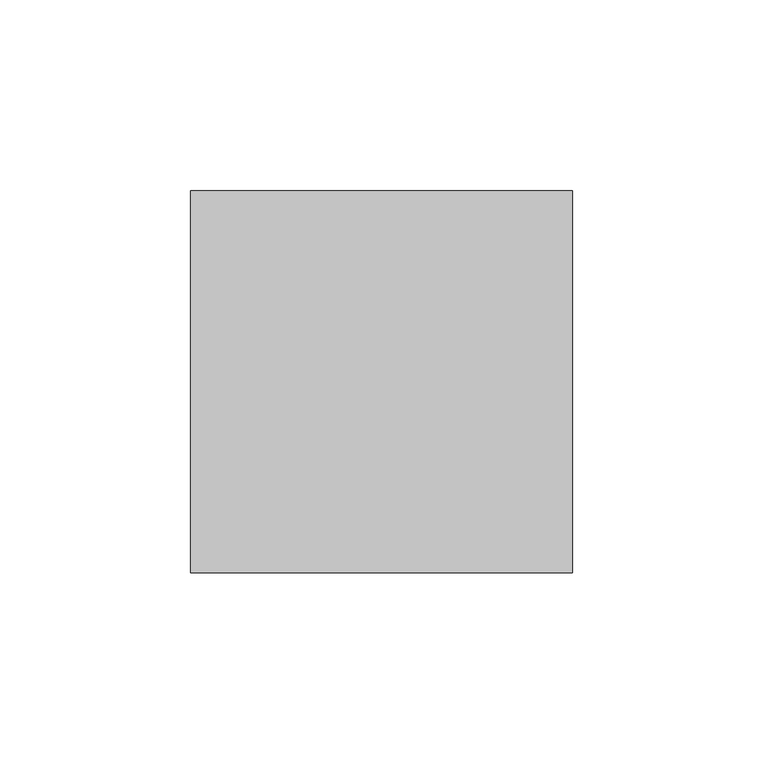
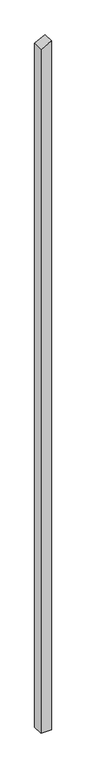
"""IFC4 building model written with IfcOpenShell, lengths in millimetres: column geometry, Holzstütze 160106 : Holzstütze 160106."""

import ifcopenshell
import ifcopenshell.guid

model = None  # the IFC model being written
_history = None  # IfcOwnerHistory: only IFC2X3 demands one
_inside = {}  # id of a spatial element -> (the spatial element, [elements in it])
_under = {}  # id of a project, library or spatial element -> (it, [spatial elements below it])
_declared = {}  # id of a project -> (the project, [libraries it declares])
_typed = {}  # id of a type object -> (the type object, [elements of that type])
_made_of = {}  # id of a material, layer set ... -> (it, [elements and type objects made of it])


def new_model(schema):
    """Start an empty IFC model of exactly this schema.

    Asked for "IFC4X3", IfcOpenShell would pick the latest addendum, in which some entities
    have other attributes; the version numbers below select the first issue.
    IFC2X3 requires an IfcOwnerHistory on every rooted entity: one is made here for all.
    """
    global model, _history
    if schema == "IFC4X3":
        model = ifcopenshell.file(schema_version=(4, 3, 0, 0))
    else:
        model = ifcopenshell.file(schema=schema)
    _inside.clear()
    _under.clear()
    _declared.clear()
    _typed.clear()
    _made_of.clear()
    _history = None
    if model.schema == "IFC2X3":
        org = make("IfcOrganization", Name="unknown")
        user = make(
            "IfcPersonAndOrganization",
            ThePerson=make("IfcPerson", FamilyName="unknown"),
            TheOrganization=org,
        )
        app = make(
            "IfcApplication",
            ApplicationDeveloper=org,
            Version="unknown",
            ApplicationFullName="unknown",
            ApplicationIdentifier="unknown",
        )
        _history = make(
            "IfcOwnerHistory",
            OwningUser=user,
            OwningApplication=app,
            ChangeAction="ADDED",
            CreationDate=0,
        )
    return model


def make(cls, **values):
    """One entity of the class cls with the attributes given. An attribute that is None is left unset."""
    return model.create_entity(
        cls, **{name: value for name, value in values.items() if value is not None}
    )


def rooted(cls, **values):
    """An entity with a GlobalId (a new one), such as an element, a storey or a relation."""
    return make(cls, GlobalId=ifcopenshell.guid.new(), OwnerHistory=_history, **values)


def si_unit(unit_type, name, prefix=None):
    """IfcSIUnit, for example si_unit("LENGTHUNIT", "METRE", prefix="MILLI")."""
    return make("IfcSIUnit", UnitType=unit_type, Prefix=prefix, Name=name)


def assignment(units):
    """IfcUnitAssignment: the units of a project."""
    return None if units is None else make("IfcUnitAssignment", Units=units)


def point(xyz):
    """IfcCartesianPoint."""
    return None if xyz is None else make("IfcCartesianPoint", Coordinates=xyz)


def direction(xyz):
    """IfcDirection."""
    return None if xyz is None else make("IfcDirection", DirectionRatios=xyz)


def frame(location, z_axis=None, x_axis=None):
    """IfcAxis2Placement3D, a coordinate frame: its origin and axes. An axis left out is left unset."""
    return make(
        "IfcAxis2Placement3D",
        Location=point(location),
        Axis=direction(z_axis),
        RefDirection=direction(x_axis),
    )


def origin():
    """The frame at (0, 0, 0) with its axes left unset."""
    return frame((0.0, 0.0, 0.0))


def place(relative_to, where):
    """IfcLocalPlacement: puts the frame where relative to a parent placement (None: the world)."""
    return make(
        "IfcLocalPlacement", PlacementRelTo=relative_to, RelativePlacement=where
    )


def context(
    kind, dimensions, precision=None, world=None, true_north=None, identifier=None
):
    """IfcGeometricRepresentationContext, for example the 3D "Model" context."""
    return make(
        "IfcGeometricRepresentationContext",
        ContextIdentifier=identifier,
        ContextType=kind,
        CoordinateSpaceDimension=dimensions,
        Precision=precision,
        WorldCoordinateSystem=world,
        TrueNorth=true_north,
    )


def project(units=None, contexts=None):
    """IfcProject with its units and contexts."""
    return rooted(
        "IfcProject",
        Name="project",
        RepresentationContexts=contexts,
        UnitsInContext=assignment(units),
    )


def spatial(cls, under=None, at=None, **own):
    """A site, building, storey or space (cls), placed at a placement, below another one or the project."""
    s = rooted(cls, ObjectPlacement=at, **own)
    if under is not None:
        _under.setdefault(under.id(), (under, []))[1].append(s)
    return s


def polyline(points):
    """IfcPolyline through the points."""
    return make("IfcPolyline", Points=[point(p) for p in points])


def outline(outer, holes=None, kind="AREA"):
    """IfcArbitraryClosedProfileDef: a profile drawn as a closed curve; with holes, ...WithVoids."""
    if holes is None:
        return make("IfcArbitraryClosedProfileDef", ProfileType=kind, OuterCurve=outer)
    return make(
        "IfcArbitraryProfileDefWithVoids",
        ProfileType=kind,
        OuterCurve=outer,
        InnerCurves=holes,
    )


def extrude(swept, where, along, depth):
    """IfcExtrudedAreaSolid: the profile swept, set in the frame where, extruded along a direction by depth."""
    return make(
        "IfcExtrudedAreaSolid",
        SweptArea=swept,
        Position=where,
        ExtrudedDirection=direction(along),
        Depth=depth,
    )


def shape(context_of_items, identifier, shape_type, items):
    """IfcShapeRepresentation: the items that make up one representation, for example the "Body"."""
    return make(
        "IfcShapeRepresentation",
        ContextOfItems=context_of_items,
        RepresentationIdentifier=identifier,
        RepresentationType=shape_type,
        Items=items,
    )


def source(mapping_origin, context_of_items, identifier, shape_type, items):
    """IfcRepresentationMap: a shape defined once, which mapped items show again and again."""
    return make(
        "IfcRepresentationMap",
        MappingOrigin=mapping_origin,
        MappedRepresentation=shape(context_of_items, identifier, shape_type, items),
    )


def transform(
    local_origin,
    x_axis=None,
    y_axis=None,
    z_axis=None,
    scale=None,
    scale2=None,
    scale3=None,
    uniform=True,
):
    """IfcCartesianTransformationOperator3D, or its non-uniform kind. x_axis, y_axis, z_axis: its Axis1, 2, 3."""
    if uniform:
        return make(
            "IfcCartesianTransformationOperator3D",
            Axis1=direction(x_axis),
            Axis2=direction(y_axis),
            LocalOrigin=point(local_origin),
            Scale=scale,
            Axis3=direction(z_axis),
        )
    return make(
        "IfcCartesianTransformationOperator3DnonUniform",
        Axis1=direction(x_axis),
        Axis2=direction(y_axis),
        LocalOrigin=point(local_origin),
        Scale=scale,
        Axis3=direction(z_axis),
        Scale2=scale2,
        Scale3=scale3,
    )


def mapped(mapping_source, mapping_target):
    """IfcMappedItem: shows the shape of a source again, moved by a transform."""
    return make(
        "IfcMappedItem", MappingSource=mapping_source, MappingTarget=mapping_target
    )


def made_of(thing, what):
    """Note that an element or type object is made of a material, layer set ...; save() writes the relation."""
    if what is not None:
        _made_of.setdefault(what.id(), (what, []))[1].append(thing)
    return thing


def element(
    cls,
    number,
    at=None,
    inside=None,
    cuts=None,
    type_object=None,
    material=None,
    context=None,
    identifier="Body",
    shape_type=None,
    held_by="IfcProductDefinitionShape",
    body=None,
    shapes=None,
    **own,
):
    """One element of the class cls, such as IfcWall. Its Tag is "e" and its number.

    at: its placement. inside: the storey or other place that contains it. cuts: it is an
    opening in that element (IfcRelVoidsElement). A single representation is given by context,
    identifier, shape_type and body (its items); several are given by shapes. held_by: the class
    of the entity that holds the representations. save() writes the other relations.
    """
    e = rooted(cls, Tag="e%d" % number, ObjectPlacement=at, **own)
    if body is not None:
        shapes = [shape(context, identifier, shape_type, body)]
    if shapes is not None:
        e.Representation = make(held_by, Representations=shapes)
    if inside is not None:
        _inside.setdefault(inside.id(), (inside, []))[1].append(e)
    if cuts is not None:
        rooted(
            "IfcRelVoidsElement", RelatingBuildingElement=cuts, RelatedOpeningElement=e
        )
    if type_object is not None:
        _typed.setdefault(type_object.id(), (type_object, []))[1].append(e)
    return made_of(e, material)


def aggregate(whole, parts):
    """IfcRelAggregates: a whole, such as a stair, and the parts it consists of."""
    return rooted("IfcRelAggregates", RelatingObject=whole, RelatedObjects=parts)


def save(model, path):
    """Write the relations noted so far, then the file.

    IfcRelAggregates (storeys below a building ...), IfcRelContainedInSpatialStructure (elements
    in a storey), IfcRelDefinesByType, IfcRelAssociatesMaterial and IfcRelDeclares: one each for
    every whole, place, type object, material and project.
    """
    for whole, parts in _under.values():
        aggregate(whole, parts)
    for where, things in _inside.values():
        rooted(
            "IfcRelContainedInSpatialStructure",
            RelatedElements=things,
            RelatingStructure=where,
        )
    for kind, things in _typed.values():
        rooted("IfcRelDefinesByType", RelatedObjects=things, RelatingType=kind)
    for what, things in _made_of.values():
        rooted("IfcRelAssociatesMaterial", RelatedObjects=things, RelatingMaterial=what)
    for by, libraries in _declared.values():
        rooted("IfcRelDeclares", RelatingContext=by, RelatedDefinitions=libraries)
    model.write(path)


def column_380c84c3(model_context):
    return source(origin(), model_context, "Body", "SweptSolid", [
        extrude(outline(polyline([(-500.0, 157297.7593015), (-500.0, 157397.7593015), (6396.6643707, 157397.7593015), (6345.7118258, 157297.7593015), (-500.0, 157297.7593015)])), frame((0.0, 33138.3551606, 0.0), z_axis=(0.0, 1.0, 0.0), x_axis=(0.0, 0.0, 1.0)), (0.0, 0.0, 1.0), 100.0),
    ])


if __name__ == "__main__":
    model = new_model("IFC4")
    model_context = context("Model", 3, world=origin())
    ifc_project = project(units=[si_unit("LENGTHUNIT", "METRE", prefix="MILLI")], contexts=[model_context])
    site = spatial("IfcSite", under=ifc_project)
    building = spatial("IfcBuilding", under=site)
    placement = place(None, origin())
    column_shape = column_380c84c3(model_context)
    element("IfcColumn", 1, ObjectType="Holzstütze 160106 : Holzstütze 160106", at=placement, inside=building, context=model_context, shape_type="MappedRepresentation", body=[
        mapped(column_shape, transform((0.0, 0.0, 0.0), x_axis=(1.0, 0.0, 0.0), y_axis=(0.0, 1.0, 0.0), z_axis=(0.0, 0.0, 1.0))),
    ])
    save(model, "model.ifc")

# Revit data of these elements
# Type "Holzstütze 160106 : Holzstütze 160106"
#   Abrechnungsart = "m"
#   Allright_Bauteil_ID = "0152St 0000143342"
#   Bezeichnung = "Holzstütze"
#   Codetext = "ST-HOLZ\\"
#   Gewerk = "Zimmer- und Holzbauarbeiten"
#   Material = "Holz"
#   Objektname = "Stütze"
#   NameOverride = "Holzstütze"
#   Reference = "Holzstütze"
#   Status = "NEW"
#   ThermalTransmittance = 0.0000 BTU/(h·ft²·°F)
#   Roll = 0.00°
#   Slope = 0.00°
#   2D Interaktion = yes
#   IsExternal = yes
#   LoadBearing = yes
# Element 1 (IfcColumn, "Holzstütze 160106 : Holzstütze 160106")
#   Materials on its faces: "holzschalung"
# Materials
#   "holzschalung": class "Unassigned", colour RGB 128 128 128, transparency 0
